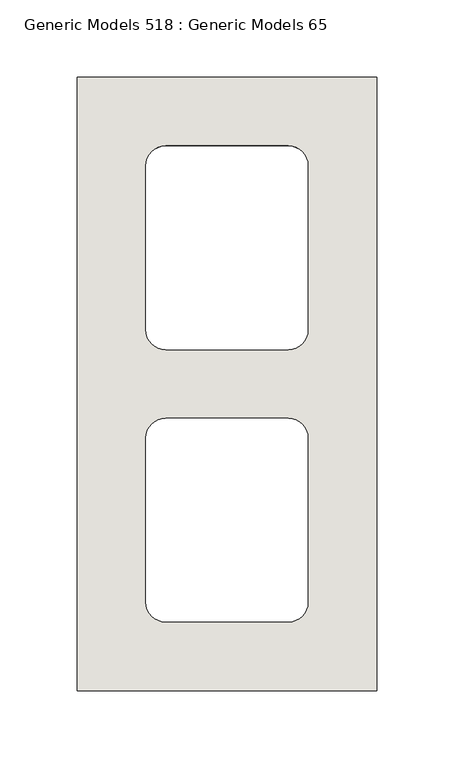
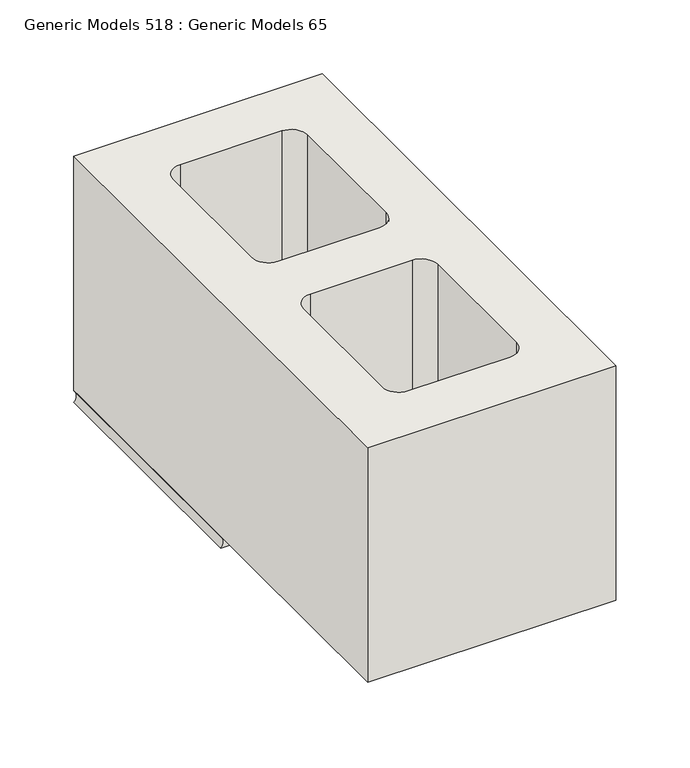
"""IFC4 building model written with IfcOpenShell, lengths in millimetres: wall geometry, Generic Models 518 : Generic Models 65."""

from ifc_helpers import new_model, si_unit, point, frame, frame_2d, origin, place, context, project, spatial, polyline, circle_curve, trimmed, segment, composite_curve, outline, extrude, source, transform, mapped, element, save
from ifc_brep_helpers import plane_surface, revolved_surface, advanced_brep


def generic_models_518_generic_models_65_b180a8d9(model_context):
    return source(origin(), model_context, "Body", "SolidModel", [
        advanced_brep(
        [(428979.0125, 503.2375, 1228.725), (428785.3375, 503.2375, 1228.725), (428785.3375, 503.2375, 1219.2), (428979.0125, 503.2375, 1219.2), (428979.0125, 701.675, 1228.725), (428979.0125, 701.675, 1219.2), (428785.3375, 701.675, 1219.2), (428785.3375, 701.675, 1228.725), (428934.5625, 538.1625, 1228.725), (428921.8625, 525.4625, 1228.725), (428842.4875, 525.4625, 1228.725), (428829.7875, 538.1625, 1228.725), (428829.7875, 644.525, 1228.725), (428842.4875, 657.225, 1228.725), (428921.8625, 657.225, 1228.725), (428934.5625, 644.525, 1228.725), (428921.8625, 525.4625, 1219.2), (428934.5625, 538.1625, 1219.2), (428842.4875, 525.4625, 1219.2), (428829.7875, 538.1625, 1219.2), (428829.7875, 644.525, 1219.2), (428842.4875, 657.225, 1219.2), (428921.8625, 657.225, 1219.2), (428934.5625, 644.525, 1219.2)],
        [
            (0, 1),
            (1, 2, circle_curve(frame((428780.4545028, 503.2375, 1223.9625), z_axis=(0.0, 1.0, 0.0), x_axis=(1.0, 0.0, 0.0)), 6.8209287)),
            (2, 3),
            (3, 0, circle_curve(frame((428983.8954972, 503.2375, 1223.9625), z_axis=(0.0, 1.0, 0.0), x_axis=(-1.0, 0.0, 0.0)), 6.8209287)),
            (4, 5, circle_curve(frame((428983.8954972, 701.675, 1223.9625), z_axis=(0.0, -1.0, 0.0), x_axis=(-1.0, 0.0, 0.0)), 6.8209287)),
            (5, 6),
            (6, 7, circle_curve(frame((428780.4545028, 701.675, 1223.9625), z_axis=(0.0, -1.0, 0.0), x_axis=(1.0, 0.0, 0.0)), 6.8209287)),
            (7, 4),
            (0, 4),
            (7, 1),
            (8, 9, circle_curve(frame((428921.8625, 538.1625, 1228.725), z_axis=(0.0, 0.0, -1.0), x_axis=(-1.0, 0.0, 0.0)), 12.7)),
            (9, 10),
            (10, 11, circle_curve(frame((428842.4875, 538.1625, 1228.725), z_axis=(0.0, 0.0, -1.0), x_axis=(-1.0, 0.0, 0.0)), 12.7)),
            (11, 12),
            (12, 13, circle_curve(frame((428842.4875, 644.525, 1228.725), z_axis=(0.0, 0.0, -1.0), x_axis=(-1.0, 0.0, 0.0)), 12.7)),
            (13, 14),
            (14, 15, circle_curve(frame((428921.8625, 644.525, 1228.725), z_axis=(0.0, 0.0, -1.0), x_axis=(-1.0, 0.0, 0.0)), 12.7)),
            (15, 8),
            (16, 9),
            (8, 17),
            (17, 16, circle_curve(frame((428921.8625, 538.1625, 1219.2), z_axis=(0.0, 0.0, -1.0), x_axis=(-1.0, 0.0, 0.0)), 12.7)),
            (16, 18),
            (18, 10),
            (18, 19, circle_curve(frame((428842.4875, 538.1625, 1219.2), z_axis=(0.0, 0.0, -1.0), x_axis=(-1.0, 0.0, 0.0)), 12.7)),
            (19, 11),
            (19, 20),
            (20, 12),
            (20, 21, circle_curve(frame((428842.4875, 644.525, 1219.2), z_axis=(0.0, 0.0, -1.0), x_axis=(-1.0, 0.0, 0.0)), 12.7)),
            (21, 13),
            (21, 22),
            (22, 14),
            (22, 23, circle_curve(frame((428921.8625, 644.525, 1219.2), z_axis=(0.0, 0.0, -1.0), x_axis=(-1.0, 0.0, 0.0)), 12.7)),
            (23, 15),
            (23, 17),
            (6, 2),
            (5, 3),
        ],
        [
            plane_surface(frame((428882.175, 503.2375, 1229.121875), z_axis=(0.0, -1.0, 0.0), x_axis=(0.0, 0.0, 1.0))),
            plane_surface(frame((428882.175, 701.675, 1229.121875), z_axis=(0.0, 1.0, 0.0), x_axis=(0.0, 0.0, 1.0))),
            plane_surface(frame((428979.0125, 503.2375, 1228.725), z_axis=(0.0, 0.0, 1.0), x_axis=(0.0, 1.0, 0.0))),
            revolved_surface(polyline([(428909.1625, 538.1625, 1228.725), (428909.1625, 538.1625, 1219.2)]), (428921.8625, 538.1625, 1412.875), (0.0, 0.0, 1.0)),
            plane_surface(frame((428842.4875, 525.4625, 1412.875), z_axis=(0.0, 1.0, 0.0), x_axis=(0.0, 0.0, -1.0))),
            revolved_surface(polyline([(428829.7875, 538.1625, 1228.725), (428829.7875, 538.1625, 1219.2)]), (428842.4875, 538.1625, 1412.875), (0.0, 0.0, 1.0)),
            plane_surface(frame((428829.7875, 644.525, 1412.875), z_axis=(1.0, 0.0, 0.0), x_axis=(0.0, 0.0, -1.0))),
            revolved_surface(polyline([(428829.7875, 644.525, 1228.725), (428829.7875, 644.525, 1219.2)]), (428842.4875, 644.525, 1412.875), (0.0, 0.0, 1.0)),
            plane_surface(frame((428921.8625, 657.225, 1412.875), z_axis=(0.0, -1.0, 0.0), x_axis=(0.0, 0.0, -1.0))),
            revolved_surface(polyline([(428909.1625, 644.525, 1228.725), (428909.1625, 644.525, 1219.2)]), (428921.8625, 644.525, 1412.875), (0.0, 0.0, 1.0)),
            plane_surface(frame((428934.5625, 538.1625, 1412.875), z_axis=(-1.0, 0.0, 0.0), x_axis=(0.0, 0.0, -1.0))),
            revolved_surface(polyline([(428787.2754315, 701.675, 1223.9625), (428787.2754315, 503.2375, 1223.9625)]), (428780.4545028, 503.2375, 1223.9625), (0.0, 1.0, 0.0)),
            plane_surface(frame((428785.3375, 503.2375, 1219.2), z_axis=(0.0, 0.0, -1.0), x_axis=(0.0, 1.0, 0.0))),
            revolved_surface(polyline([(428977.07456850004, 701.675, 1223.9625), (428977.07456850004, 503.2375, 1223.9625)]), (428983.8954972, 503.2375, 1223.9625), (0.0, 1.0, 0.0)),
        ],
        [
            (0, [[1, 2, 3, 4]]),
            (1, [[5, 6, 7, 8]]),
            (2, [[-1, 9, -8, 10], [11, 12, 13, 14, 15, 16, 17, 18]]),
            (3, [[19, -11, 20, 21]]),
            (4, [[-19, 22, 23, -12]]),
            (5, [[-23, 24, 25, -13]]),
            (6, [[-25, 26, 27, -14]]),
            (7, [[-27, 28, 29, -15]]),
            (8, [[-29, 30, 31, -16]]),
            (9, [[-31, 32, 33, -17]]),
            (10, [[-33, 34, -20, -18]]),
            (11, [[-2, -10, -7, 35]]),
            (12, [[-3, -35, -6, 36], [-21, -34, -32, -30, -28, -26, -24, -22]]),
            (13, [[-4, -36, -5, -9]]),
        ],
    ),
        extrude(outline(polyline([(428979.0125, 304.8), (428785.3375, 304.8), (428785.3375, 701.675), (428979.0125, 701.675), (428979.0125, 304.8)]), holes=[composite_curve([segment(polyline([(428934.5625, 538.1625), (428934.5625, 644.525)]), True, "CONTINUOUS"), segment(trimmed(circle_curve(frame_2d((428921.8625, 644.525)), 12.7), [point((428934.5625, 644.525))], [point((428921.8625, 657.225))], True, "CARTESIAN"), True, "CONTINUOUS"), segment(polyline([(428921.8625, 657.225), (428842.4875, 657.225)]), True, "CONTINUOUS"), segment(trimmed(circle_curve(frame_2d((428842.4875, 644.525)), 12.7), [point((428842.4875, 657.225))], [point((428829.7875, 644.525))], True, "CARTESIAN"), True, "CONTINUOUS"), segment(polyline([(428829.7875, 644.525), (428829.7875, 538.1625)]), True, "CONTINUOUS"), segment(trimmed(circle_curve(frame_2d((428842.4875, 538.1625)), 12.7), [point((428829.7875, 538.1625))], [point((428842.4875, 525.4625))], True, "CARTESIAN"), True, "CONTINUOUS"), segment(polyline([(428842.4875, 525.4625), (428921.8625, 525.4625)]), True, "CONTINUOUS"), segment(trimmed(circle_curve(frame_2d((428921.8625, 538.1625)), 12.7), [point((428921.8625, 525.4625))], [point((428934.5625, 538.1625))], True, "CARTESIAN"), True, "CONTINUOUS")], self_intersect=False), composite_curve([segment(polyline([(428829.7875, 468.3125), (428829.7875, 361.95)]), True, "CONTINUOUS"), segment(trimmed(circle_curve(frame_2d((428842.4875, 361.95)), 12.7), [point((428829.7875, 361.95))], [point((428842.4875, 349.25))], True, "CARTESIAN"), True, "CONTINUOUS"), segment(polyline([(428842.4875, 349.25), (428921.8625, 349.25)]), True, "CONTINUOUS"), segment(trimmed(circle_curve(frame_2d((428921.8625, 361.95)), 12.7), [point((428921.8625, 349.25))], [point((428934.5625, 361.95))], True, "CARTESIAN"), True, "CONTINUOUS"), segment(polyline([(428934.5625, 361.95), (428934.5625, 468.3125)]), True, "CONTINUOUS"), segment(trimmed(circle_curve(frame_2d((428921.8625, 468.3125)), 12.7), [point((428934.5625, 468.3125))], [point((428921.8625, 481.0125))], True, "CARTESIAN"), True, "CONTINUOUS"), segment(polyline([(428921.8625, 481.0125), (428842.4875, 481.0125)]), True, "CONTINUOUS"), segment(trimmed(circle_curve(frame_2d((428842.4875, 468.3125)), 12.7), [point((428842.4875, 481.0125))], [point((428829.7875, 468.3125))], True, "CARTESIAN"), True, "CONTINUOUS")], self_intersect=False)]), frame((0.0, 0.0, 1228.725), z_axis=(0.0, 0.0, 1.0), x_axis=(1.0, 0.0, 0.0)), (0.0, 0.0, 1.0), 193.675),
    ])


if __name__ == "__main__":
    model = new_model("IFC4")
    model_context = context("Model", 3, world=origin())
    ifc_project = project(units=[si_unit("LENGTHUNIT", "METRE", prefix="MILLI")], contexts=[model_context])
    site = spatial("IfcSite", under=ifc_project)
    building = spatial("IfcBuilding", under=site)
    placement = place(None, origin())
    generic_models_518_generic_models_65_shape = generic_models_518_generic_models_65_b180a8d9(model_context)
    element("IfcWall", 1, ObjectType="Generic Models 518 : Generic Models 65", at=placement, inside=building, context=model_context, shape_type="MappedRepresentation", body=[
        mapped(generic_models_518_generic_models_65_shape, transform((0.0, 0.0, 0.0), x_axis=(1.0, 0.0, 0.0), y_axis=(0.0, 1.0, 0.0), z_axis=(0.0, 0.0, 1.0))),
    ])
    save(model, "model.ifc")

# Revit data of these elements
# Element 1 (IfcWall, "Generic Models 518 : Generic Models 65")
#   Materials on its faces: "CMU (SEE 'WALL TAG' FOR SIZE)", "MORTAR JOINT"
# Materials
#   "CMU (SEE 'WALL TAG' FOR SIZE)": class "Masonry", colour RGB 203 203 199, transparency 0, Description = "Concrete masonry units", Cost = 0
#   "MORTAR JOINT": class "Generic", colour RGB 120 120 120, transparency 0, Cost = 0
